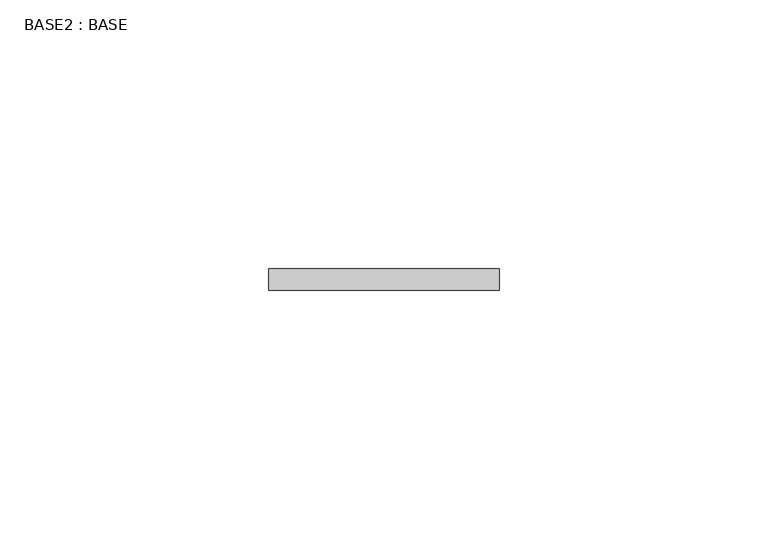
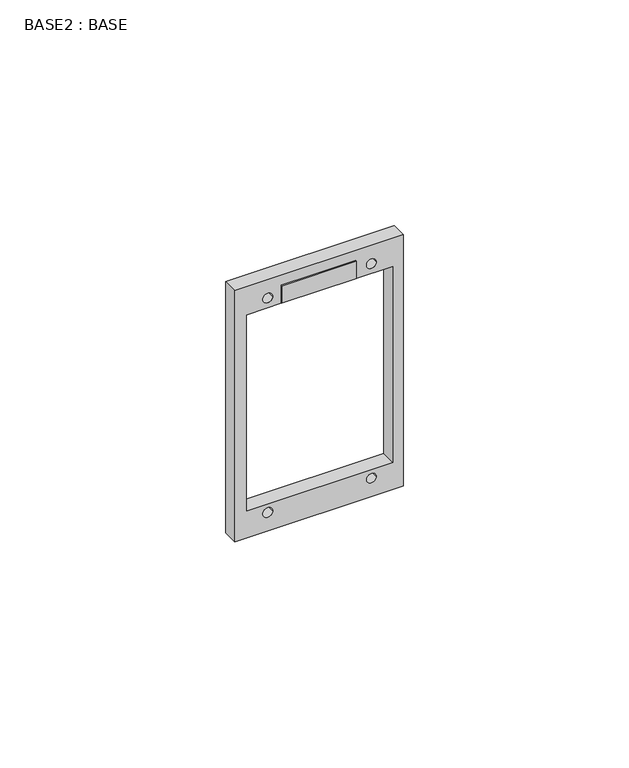
"""IFC4 building model written with IfcOpenShell, lengths in millimetres: proxy geometry, BASE2 : BASE."""

import ifcopenshell
import ifcopenshell.guid

model = None  # the IFC model being written
_history = None  # IfcOwnerHistory: only IFC2X3 demands one
_inside = {}  # id of a spatial element -> (the spatial element, [elements in it])
_under = {}  # id of a project, library or spatial element -> (it, [spatial elements below it])
_declared = {}  # id of a project -> (the project, [libraries it declares])
_typed = {}  # id of a type object -> (the type object, [elements of that type])
_made_of = {}  # id of a material, layer set ... -> (it, [elements and type objects made of it])


def new_model(schema):
    """Start an empty IFC model of exactly this schema.

    Asked for "IFC4X3", IfcOpenShell would pick the latest addendum, in which some entities
    have other attributes; the version numbers below select the first issue.
    IFC2X3 requires an IfcOwnerHistory on every rooted entity: one is made here for all.
    """
    global model, _history
    if schema == "IFC4X3":
        model = ifcopenshell.file(schema_version=(4, 3, 0, 0))
    else:
        model = ifcopenshell.file(schema=schema)
    _inside.clear()
    _under.clear()
    _declared.clear()
    _typed.clear()
    _made_of.clear()
    _history = None
    if model.schema == "IFC2X3":
        org = make("IfcOrganization", Name="unknown")
        user = make(
            "IfcPersonAndOrganization",
            ThePerson=make("IfcPerson", FamilyName="unknown"),
            TheOrganization=org,
        )
        app = make(
            "IfcApplication",
            ApplicationDeveloper=org,
            Version="unknown",
            ApplicationFullName="unknown",
            ApplicationIdentifier="unknown",
        )
        _history = make(
            "IfcOwnerHistory",
            OwningUser=user,
            OwningApplication=app,
            ChangeAction="ADDED",
            CreationDate=0,
        )
    return model


def make(cls, **values):
    """One entity of the class cls with the attributes given. An attribute that is None is left unset."""
    return model.create_entity(
        cls, **{name: value for name, value in values.items() if value is not None}
    )


def rooted(cls, **values):
    """An entity with a GlobalId (a new one), such as an element, a storey or a relation."""
    return make(cls, GlobalId=ifcopenshell.guid.new(), OwnerHistory=_history, **values)


def si_unit(unit_type, name, prefix=None):
    """IfcSIUnit, for example si_unit("LENGTHUNIT", "METRE", prefix="MILLI")."""
    return make("IfcSIUnit", UnitType=unit_type, Prefix=prefix, Name=name)


def assignment(units):
    """IfcUnitAssignment: the units of a project."""
    return None if units is None else make("IfcUnitAssignment", Units=units)


def point(xyz):
    """IfcCartesianPoint."""
    return None if xyz is None else make("IfcCartesianPoint", Coordinates=xyz)


def direction(xyz):
    """IfcDirection."""
    return None if xyz is None else make("IfcDirection", DirectionRatios=xyz)


def frame(location, z_axis=None, x_axis=None):
    """IfcAxis2Placement3D, a coordinate frame: its origin and axes. An axis left out is left unset."""
    return make(
        "IfcAxis2Placement3D",
        Location=point(location),
        Axis=direction(z_axis),
        RefDirection=direction(x_axis),
    )


def frame_2d(location, x_axis=None):
    """IfcAxis2Placement2D, a coordinate frame in the plane: its origin and x axis."""
    return make(
        "IfcAxis2Placement2D", Location=point(location), RefDirection=direction(x_axis)
    )


def origin():
    """The frame at (0, 0, 0) with its axes left unset."""
    return frame((0.0, 0.0, 0.0))


def place(relative_to, where):
    """IfcLocalPlacement: puts the frame where relative to a parent placement (None: the world)."""
    return make(
        "IfcLocalPlacement", PlacementRelTo=relative_to, RelativePlacement=where
    )


def context(
    kind, dimensions, precision=None, world=None, true_north=None, identifier=None
):
    """IfcGeometricRepresentationContext, for example the 3D "Model" context."""
    return make(
        "IfcGeometricRepresentationContext",
        ContextIdentifier=identifier,
        ContextType=kind,
        CoordinateSpaceDimension=dimensions,
        Precision=precision,
        WorldCoordinateSystem=world,
        TrueNorth=true_north,
    )


def project(units=None, contexts=None):
    """IfcProject with its units and contexts."""
    return rooted(
        "IfcProject",
        Name="project",
        RepresentationContexts=contexts,
        UnitsInContext=assignment(units),
    )


def spatial(cls, under=None, at=None, **own):
    """A site, building, storey or space (cls), placed at a placement, below another one or the project."""
    s = rooted(cls, ObjectPlacement=at, **own)
    if under is not None:
        _under.setdefault(under.id(), (under, []))[1].append(s)
    return s


def polyline(points):
    """IfcPolyline through the points."""
    return make("IfcPolyline", Points=[point(p) for p in points])


def circle_curve(where, radius):
    """IfcCircle in the frame where."""
    return make("IfcCircle", Position=where, Radius=radius)


def trimmed(basis, trim1, trim2, sense, master):
    """IfcTrimmedCurve: the piece of a basis curve between two trims."""
    return make(
        "IfcTrimmedCurve",
        BasisCurve=basis,
        Trim1=trim1,
        Trim2=trim2,
        SenseAgreement=sense,
        MasterRepresentation=master,
    )


def segment(curve, same_sense, transition):
    """IfcCompositeCurveSegment."""
    return make(
        "IfcCompositeCurveSegment",
        Transition=transition,
        SameSense=same_sense,
        ParentCurve=curve,
    )


def composite_curve(segments, self_intersect=None):
    """IfcCompositeCurve: segments joined end to end."""
    return make("IfcCompositeCurve", Segments=segments, SelfIntersect=self_intersect)


def outline(outer, holes=None, kind="AREA"):
    """IfcArbitraryClosedProfileDef: a profile drawn as a closed curve; with holes, ...WithVoids."""
    if holes is None:
        return make("IfcArbitraryClosedProfileDef", ProfileType=kind, OuterCurve=outer)
    return make(
        "IfcArbitraryProfileDefWithVoids",
        ProfileType=kind,
        OuterCurve=outer,
        InnerCurves=holes,
    )


def extrude(swept, where, along, depth):
    """IfcExtrudedAreaSolid: the profile swept, set in the frame where, extruded along a direction by depth."""
    return make(
        "IfcExtrudedAreaSolid",
        SweptArea=swept,
        Position=where,
        ExtrudedDirection=direction(along),
        Depth=depth,
    )


def shape(context_of_items, identifier, shape_type, items):
    """IfcShapeRepresentation: the items that make up one representation, for example the "Body"."""
    return make(
        "IfcShapeRepresentation",
        ContextOfItems=context_of_items,
        RepresentationIdentifier=identifier,
        RepresentationType=shape_type,
        Items=items,
    )


def source(mapping_origin, context_of_items, identifier, shape_type, items):
    """IfcRepresentationMap: a shape defined once, which mapped items show again and again."""
    return make(
        "IfcRepresentationMap",
        MappingOrigin=mapping_origin,
        MappedRepresentation=shape(context_of_items, identifier, shape_type, items),
    )


def transform(
    local_origin,
    x_axis=None,
    y_axis=None,
    z_axis=None,
    scale=None,
    scale2=None,
    scale3=None,
    uniform=True,
):
    """IfcCartesianTransformationOperator3D, or its non-uniform kind. x_axis, y_axis, z_axis: its Axis1, 2, 3."""
    if uniform:
        return make(
            "IfcCartesianTransformationOperator3D",
            Axis1=direction(x_axis),
            Axis2=direction(y_axis),
            LocalOrigin=point(local_origin),
            Scale=scale,
            Axis3=direction(z_axis),
        )
    return make(
        "IfcCartesianTransformationOperator3DnonUniform",
        Axis1=direction(x_axis),
        Axis2=direction(y_axis),
        LocalOrigin=point(local_origin),
        Scale=scale,
        Axis3=direction(z_axis),
        Scale2=scale2,
        Scale3=scale3,
    )


def mapped(mapping_source, mapping_target):
    """IfcMappedItem: shows the shape of a source again, moved by a transform."""
    return make(
        "IfcMappedItem", MappingSource=mapping_source, MappingTarget=mapping_target
    )


def made_of(thing, what):
    """Note that an element or type object is made of a material, layer set ...; save() writes the relation."""
    if what is not None:
        _made_of.setdefault(what.id(), (what, []))[1].append(thing)
    return thing


def element(
    cls,
    number,
    at=None,
    inside=None,
    cuts=None,
    type_object=None,
    material=None,
    context=None,
    identifier="Body",
    shape_type=None,
    held_by="IfcProductDefinitionShape",
    body=None,
    shapes=None,
    **own,
):
    """One element of the class cls, such as IfcWall. Its Tag is "e" and its number.

    at: its placement. inside: the storey or other place that contains it. cuts: it is an
    opening in that element (IfcRelVoidsElement). A single representation is given by context,
    identifier, shape_type and body (its items); several are given by shapes. held_by: the class
    of the entity that holds the representations. save() writes the other relations.
    """
    e = rooted(cls, Tag="e%d" % number, ObjectPlacement=at, **own)
    if body is not None:
        shapes = [shape(context, identifier, shape_type, body)]
    if shapes is not None:
        e.Representation = make(held_by, Representations=shapes)
    if inside is not None:
        _inside.setdefault(inside.id(), (inside, []))[1].append(e)
    if cuts is not None:
        rooted(
            "IfcRelVoidsElement", RelatingBuildingElement=cuts, RelatedOpeningElement=e
        )
    if type_object is not None:
        _typed.setdefault(type_object.id(), (type_object, []))[1].append(e)
    return made_of(e, material)


def aggregate(whole, parts):
    """IfcRelAggregates: a whole, such as a stair, and the parts it consists of."""
    return rooted("IfcRelAggregates", RelatingObject=whole, RelatedObjects=parts)


def save(model, path):
    """Write the relations noted so far, then the file.

    IfcRelAggregates (storeys below a building ...), IfcRelContainedInSpatialStructure (elements
    in a storey), IfcRelDefinesByType, IfcRelAssociatesMaterial and IfcRelDeclares: one each for
    every whole, place, type object, material and project.
    """
    for whole, parts in _under.values():
        aggregate(whole, parts)
    for where, things in _inside.values():
        rooted(
            "IfcRelContainedInSpatialStructure",
            RelatedElements=things,
            RelatingStructure=where,
        )
    for kind, things in _typed.values():
        rooted("IfcRelDefinesByType", RelatedObjects=things, RelatingType=kind)
    for what, things in _made_of.values():
        rooted("IfcRelAssociatesMaterial", RelatedObjects=things, RelatingMaterial=what)
    for by, libraries in _declared.values():
        rooted("IfcRelDeclares", RelatingContext=by, RelatedDefinitions=libraries)
    model.write(path)


def base2_base_c05baaad(model_context):
    return source(origin(), model_context, "Body", "SweptSolid", [
        extrude(outline(polyline([(2465.0719295, 1293.4498458), (2465.0719295, 1291.7192449), (2446.0719295, 1291.7192449), (2446.0719295, 1293.4498458), (2465.0719295, 1293.4498458)])), frame((0.0, 0.0, 60.3), z_axis=(0.0, 0.0, 1.0), x_axis=(1.0, 0.0, 0.0)), (0.0, 0.0, 1.0), 4.7),
        extrude(outline(polyline([(0.0, 2434.0719295), (0.0, 2477.0719295), (68.0, 2477.0719295), (68.0, 2434.0719295), (0.0, 2434.0719295)]), holes=[composite_curve([segment(trimmed(circle_curve(frame_2d((63.0, 2468.9719295)), 1.25), [point((63.0, 2467.7219295))], [point((63.0, 2470.2219295))], True, "CARTESIAN"), True, "CONTINUOUS"), segment(trimmed(circle_curve(frame_2d((63.0, 2468.9719295)), 1.25), [point((63.0, 2470.2219295))], [point((63.0, 2467.7219295))], True, "CARTESIAN"), True, "CONTINUOUS")], self_intersect=False), composite_curve([segment(trimmed(circle_curve(frame_2d((5.0, 2468.9719295)), 1.25), [point((5.0, 2470.2219295))], [point((5.0, 2467.7219295))], True, "CARTESIAN"), True, "CONTINUOUS"), segment(trimmed(circle_curve(frame_2d((5.0, 2468.9719295)), 1.25), [point((5.0, 2467.7219295))], [point((5.0, 2470.2219295))], True, "CARTESIAN"), True, "CONTINUOUS")], self_intersect=False), composite_curve([segment(trimmed(circle_curve(frame_2d((5.0, 2442.4719295)), 1.25), [point((5.0, 2443.7219295))], [point((5.0, 2441.2219295))], True, "CARTESIAN"), True, "CONTINUOUS"), segment(trimmed(circle_curve(frame_2d((5.0, 2442.4719295)), 1.25), [point((5.0, 2441.2219295))], [point((5.0, 2443.7219295))], True, "CARTESIAN"), True, "CONTINUOUS")], self_intersect=False), composite_curve([segment(trimmed(circle_curve(frame_2d((63.0, 2442.4719295)), 1.25), [point((63.0, 2443.7219295))], [point((63.0, 2441.2219295))], True, "CARTESIAN"), True, "CONTINUOUS"), segment(trimmed(circle_curve(frame_2d((63.0, 2442.4719295)), 1.25), [point((63.0, 2441.2219295))], [point((63.0, 2443.7219295))], True, "CARTESIAN"), True, "CONTINUOUS")], self_intersect=False), polyline([(7.3, 2474.3719295), (7.3, 2437.0719295), (60.3, 2437.0719295), (60.3, 2446.0719295), (65.0, 2446.0719295), (65.0, 2465.0719295), (60.3, 2465.0719295), (60.3, 2474.3719295), (7.3, 2474.3719295)])]), frame((0.0, 1291.7192449, 0.0), z_axis=(0.0, 1.0, 0.0), x_axis=(0.0, 0.0, 1.0)), (0.0, 0.0, 1.0), 4.0),
    ])


if __name__ == "__main__":
    model = new_model("IFC4")
    model_context = context("Model", 3, world=origin())
    ifc_project = project(units=[si_unit("LENGTHUNIT", "METRE", prefix="MILLI")], contexts=[model_context])
    site = spatial("IfcSite", under=ifc_project)
    building = spatial("IfcBuilding", under=site)
    placement = place(None, origin())
    base2_base_shape = base2_base_c05baaad(model_context)
    element("IfcBuildingElementProxy", 1, Name="BASE2 : BASE", ObjectType="BASE2 : BASE", at=placement, inside=building, context=model_context, shape_type="MappedRepresentation", body=[
        mapped(base2_base_shape, transform((0.0, 0.0, 0.0), x_axis=(1.0, 0.0, 0.0), y_axis=(0.0, 1.0, 0.0), z_axis=(0.0, 0.0, 1.0))),
    ])
    save(model, "model.ifc")

# Revit data of these elements
# Element 1 (IfcBuildingElementProxy, "BASE2 : BASE")
#   Materials on its faces: ".BOX FUNDO"
# Materials
#   ".BOX FUNDO": class "Vidro", colour RGB 236 240 239, transparency 0.15, Cost = 0
